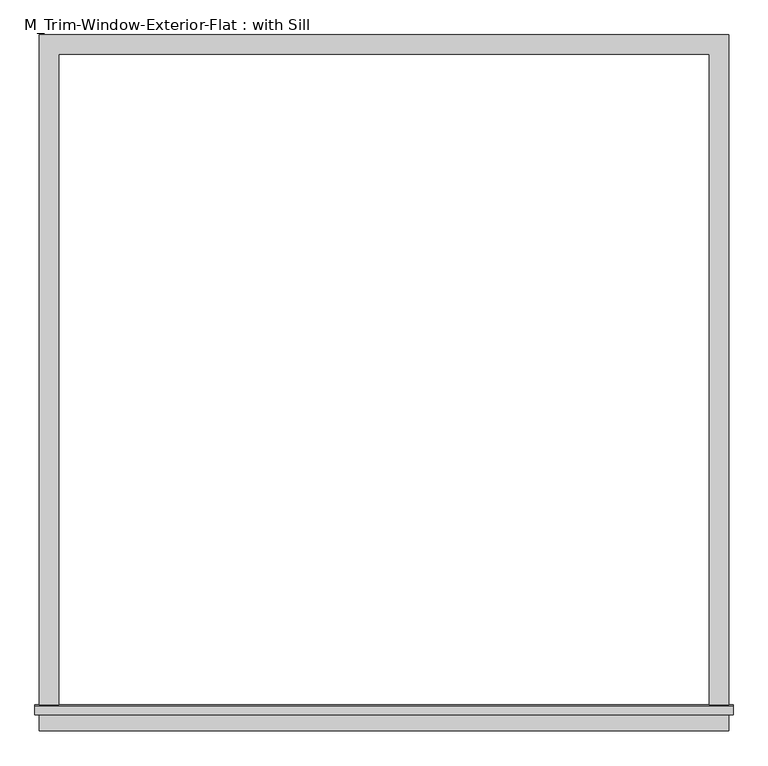
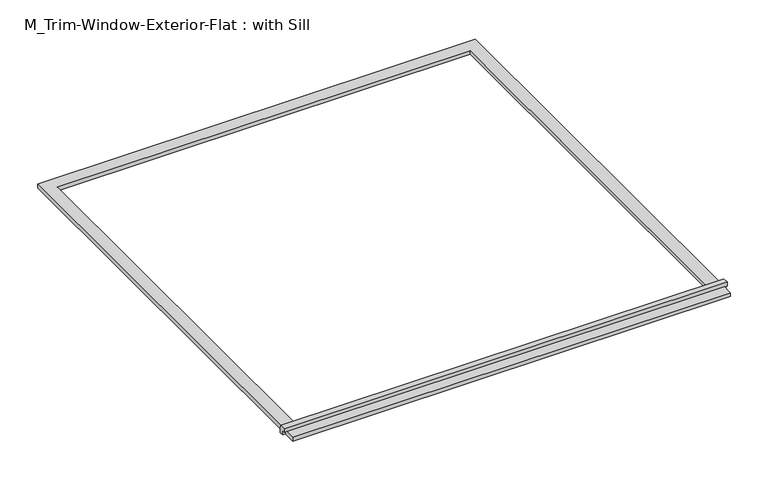
"""IFC4 building model written with IfcOpenShell, lengths in millimetres: proxy geometry, M_Trim-Window-Exterior-Flat : with Sill."""

from ifc_helpers import new_model, si_unit, frame, origin, origin_with_axes, place, context, project, spatial, polyline, outline, extrude, source, transform, mapped, element, save


def m_trim_window_exterior_flat_with_sill_08423512(model_context):
    return source(origin(), model_context, "Body", "SweptSolid", [
        extrude(outline(polyline([(1060.0, -2020.4323709), (1060.0, -2080.4323709), (-1060.0, -2080.4323709), (-1060.0, -2020.4323709), (1060.0, -2020.4323709)])), origin_with_axes(), (0.0, 0.0, 1.0), 19.05),
        extrude(outline(polyline([(-2030.0, 38.1), (-2002.4580645, 38.1), (-2000.0, 19.05), (-2000.0, 0.0), (-2020.4323709, 0.0), (-2020.4323709, 19.05), (-2030.0, 19.05), (-2030.0, 38.1)])), frame((-1072.7, 0.0, 0.0), z_axis=(1.0, 0.0, 0.0), x_axis=(0.0, 1.0, 0.0)), (0.0, 0.0, 1.0), 2145.4),
        extrude(outline(polyline([(-1060.0, 60.0), (1060.0, 60.0), (1060.0, -2000.0), (1000.0, -2000.0), (1000.0, 0.0), (-1000.0, 0.0), (-1000.0, -2000.0), (-1060.0, -2000.0), (-1060.0, 60.0)])), origin_with_axes(), (0.0, 0.0, 1.0), 19.05),
    ])


if __name__ == "__main__":
    model = new_model("IFC4")
    model_context = context("Model", 3, world=origin())
    ifc_project = project(units=[si_unit("LENGTHUNIT", "METRE", prefix="MILLI")], contexts=[model_context])
    site = spatial("IfcSite", under=ifc_project)
    building = spatial("IfcBuilding", under=site)
    placement = place(None, origin())
    m_trim_window_exterior_flat_with_sill_shape = m_trim_window_exterior_flat_with_sill_08423512(model_context)
    element("IfcBuildingElementProxy", 1, Name="M_Trim-Window-Exterior-Flat : with Sill", ObjectType="M_Trim-Window-Exterior-Flat : with Sill", at=placement, inside=building, context=model_context, shape_type="MappedRepresentation", body=[
        mapped(m_trim_window_exterior_flat_with_sill_shape, transform((0.0, 0.0, 0.0), x_axis=(1.0, 0.0, 0.0), y_axis=(0.0, 1.0, 0.0), z_axis=(0.0, 0.0, 1.0))),
    ])
    save(model, "model.ifc")

# Revit data of these elements
# Project information
#   Название организации = "Organization Name"
#   Описание организации = "Organization Description"
#   Наименование здания = "Building Name"
#   Дата утверждения проекта = "Issue Date"
#   Статус проекта = "Project Status"
#   Заказчик = "Client Name"
#   Адрес проекта = "Enter address here\nAddress Line 2"
#   Наименование проекта = "Project Name"
#   Номер проекта = "Project Number"
# Type "M_Trim-Window-Exterior-Flat : with Sill"
#   Trim Width = 60 mm
#   Trim Thickness_Picture Frame = 30 mm
#   Trim Thickness_with Sill = 19.05 mm
#   Sill Thickness = 30 mm
#   Opening Width [instance default] = 600 mm
#   Opening Height [instance default] = 900 mm
#   Default Elevation = 1200 mm
#   Sill = yes
#   Picture Frame = no
#   Trim Material [instance default] = none
# Element 1 (IfcBuildingElementProxy, "M_Trim-Window-Exterior-Flat : with Sill")
#   Opening Width = 2000 mm
#   Opening Height = 2000 mm
#   Trim Material = Clad - White
#   Materials on its faces: "Clad - White"
# Materials
#   "Clad - White": class "Wood", colour RGB 245 245 243, transparency 0, Cost = 0
